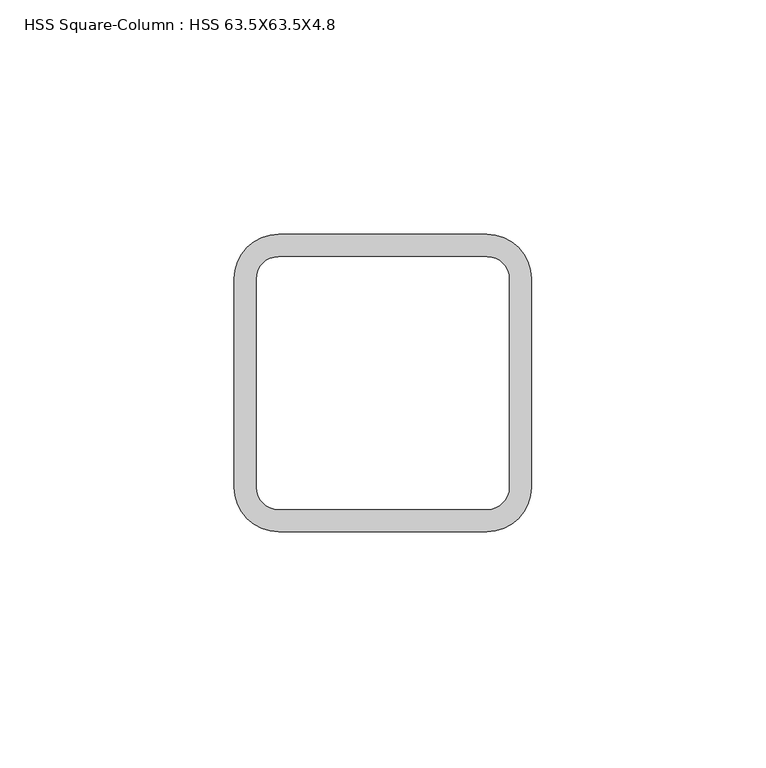
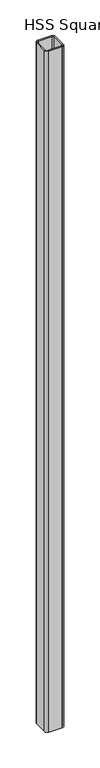
"""IFC4 building model written with IfcOpenShell, lengths in millimetres: column geometry, HSS Square-Column : HSS 63.5X63.5X4.8."""

from ifc_helpers import new_model, si_unit, point, frame, frame_2d, origin, place, context, project, spatial, polyline, circle_curve, trimmed, segment, composite_curve, outline, extrude, source, transform, mapped, element, save


def hss_square_column_hss_63_5x63_5x4_8_f9c1b5a1(model_context):
    return source(origin(), model_context, "Body", "SweptSolid", [
        extrude(outline(composite_curve([segment(trimmed(circle_curve(frame_2d((22.225, 22.225)), 9.525), [point((22.225, 31.75))], [point((31.75, 22.225))], False, "CARTESIAN"), True, "CONTINUOUS"), segment(polyline([(31.75, 22.225), (31.75, -22.225)]), True, "CONTINUOUS"), segment(trimmed(circle_curve(frame_2d((22.225, -22.225)), 9.525), [point((31.75, -22.225))], [point((22.225, -31.75))], False, "CARTESIAN"), True, "CONTINUOUS"), segment(polyline([(22.225, -31.75), (-22.225, -31.75)]), True, "CONTINUOUS"), segment(trimmed(circle_curve(frame_2d((-22.225, -22.225)), 9.525), [point((-22.225, -31.75))], [point((-31.75, -22.225))], False, "CARTESIAN"), True, "CONTINUOUS"), segment(polyline([(-31.75, -22.225), (-31.75, 22.225)]), True, "CONTINUOUS"), segment(trimmed(circle_curve(frame_2d((-22.225, 22.225)), 9.525), [point((-31.75, 22.225))], [point((-22.225, 31.75))], False, "CARTESIAN"), True, "CONTINUOUS"), segment(polyline([(-22.225, 31.75), (22.225, 31.75)]), True, "CONTINUOUS")], self_intersect=False), holes=[composite_curve([segment(polyline([(22.225, 26.9875), (-22.225, 26.9875)]), True, "CONTINUOUS"), segment(trimmed(circle_curve(frame_2d((-22.225, 22.225)), 4.7625), [point((-22.225, 26.9875))], [point((-26.9875, 22.225))], True, "CARTESIAN"), True, "CONTINUOUS"), segment(polyline([(-26.9875, 22.225), (-26.9875, -22.225)]), True, "CONTINUOUS"), segment(trimmed(circle_curve(frame_2d((-22.225, -22.225)), 4.7625), [point((-26.9875, -22.225))], [point((-22.225, -26.9875))], True, "CARTESIAN"), True, "CONTINUOUS"), segment(polyline([(-22.225, -26.9875), (22.225, -26.9875)]), True, "CONTINUOUS"), segment(trimmed(circle_curve(frame_2d((22.225, -22.225)), 4.7625), [point((22.225, -26.9875))], [point((26.9875, -22.225))], True, "CARTESIAN"), True, "CONTINUOUS"), segment(polyline([(26.9875, -22.225), (26.9875, 22.225)]), True, "CONTINUOUS"), segment(trimmed(circle_curve(frame_2d((22.225, 22.225)), 4.7625), [point((26.9875, 22.225))], [point((22.225, 26.9875))], True, "CARTESIAN"), True, "CONTINUOUS")], self_intersect=False)]), frame((0.0, 0.0, 3220.0), z_axis=(0.0, 0.0, 1.0), x_axis=(1.0, 0.0, 0.0)), (0.0, 0.0, 1.0), 2400.0),
    ])


if __name__ == "__main__":
    model = new_model("IFC4")
    model_context = context("Model", 3, world=origin())
    ifc_project = project(units=[si_unit("LENGTHUNIT", "METRE", prefix="MILLI")], contexts=[model_context])
    site = spatial("IfcSite", under=ifc_project)
    building = spatial("IfcBuilding", under=site)
    placement = place(None, origin())
    hss_square_column_hss_63_5x63_5x4_8_shape = hss_square_column_hss_63_5x63_5x4_8_f9c1b5a1(model_context)
    element("IfcColumn", 1, ObjectType="HSS Square-Column : HSS 63.5X63.5X4.8", at=placement, inside=building, context=model_context, shape_type="MappedRepresentation", body=[
        mapped(hss_square_column_hss_63_5x63_5x4_8_shape, transform((0.0, 0.0, 0.0), x_axis=(1.0, 0.0, 0.0), y_axis=(0.0, 1.0, 0.0), z_axis=(0.0, 0.0, 1.0))),
    ])
    save(model, "model.ifc")

# Revit data of these elements
# Type "HSS Square-Column : HSS 63.5X63.5X4.8"
#   Section Name Key = "HSS 2 1/2X2 1/2X3/16"
#   Assembly Code = "B10"
#   Width = 6.35 cm
#   Wall Nominal Thickness = 0.4763 cm
#   Wall Design Thickness = 0.442 cm
#   Torsional Moment of Inertia = 93.6521 cm⁴
#   Torsional Modulus = 30.4799 cm³
#   Section Area = 9.93546 cm²
#   Plastic Modulus weak axis = 21.6309 cm³
#   Plastic Modulus strong axis = 21.6309 cm³
#   Outer Fillet = 0.9525 cm
#   Nominal Weight = 8.31884 kgf/m
#   Moment of Inertia weak axis = 56.1912 cm⁴
#   Moment of Inertia strong axis = 56.1912 cm⁴
#   Inner Fillet = 0.4763 cm
#   Height = 6.35 cm
#   Elastic Modulus weak axis = 17.698 cm³
#   Elastic Modulus strong axis = 17.698 cm³
#   Centroid Vertical = 3.175 cm
#   Centroid Horizontal = 3.175 cm
#   Structural Material [instance default] = Steel ASTM A500, Grade B, Rectangular and Square
#   Principal Axes Angle = 0
# Element 1 (IfcColumn, "HSS Square-Column : HSS 63.5X63.5X4.8")
#   Structural Material = none
# Materials
#   "Steel ASTM A500, Grade B, Rectangular and Square": class "Metal", colour RGB 199 199 199, transparency 0, Description = "Carbon steel", Cost = 0
